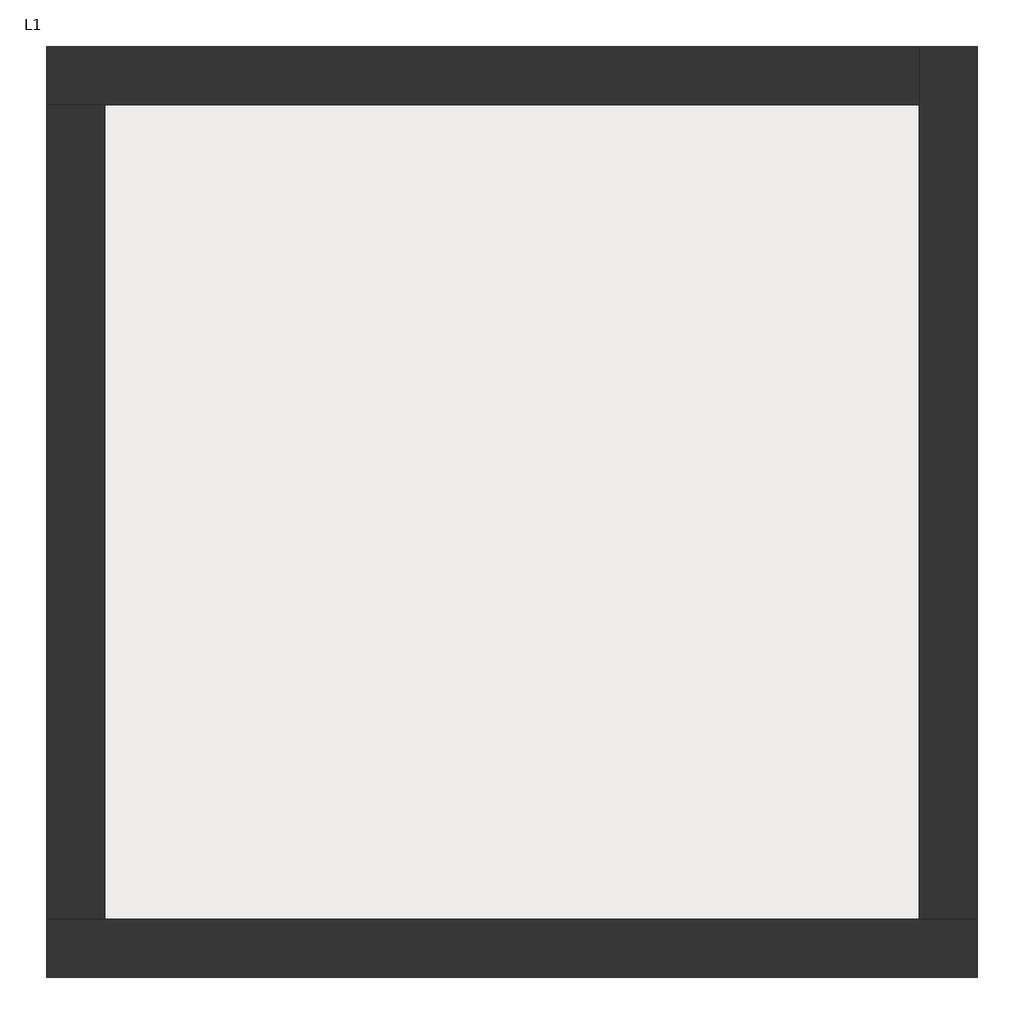
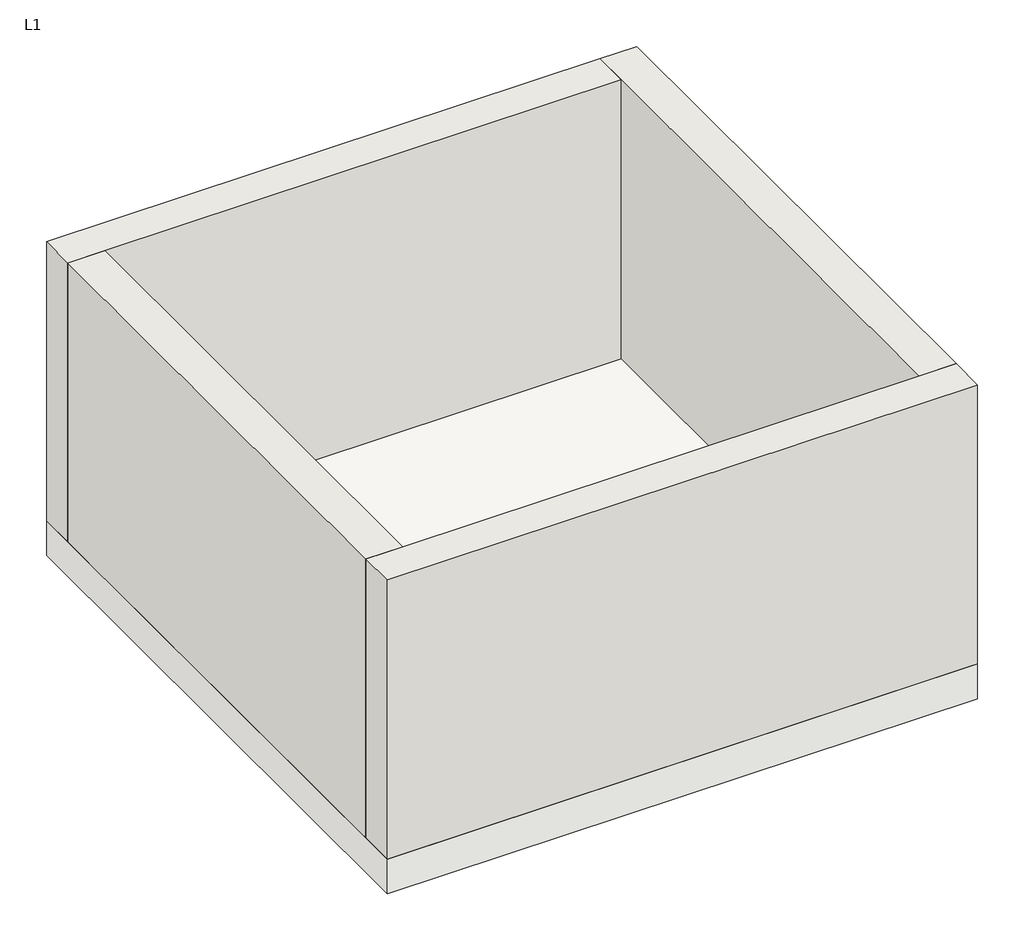
# One storey: 4 walls, 1 slab.
"""IFC4 building model written with IfcOpenShell, lengths in millimetres."""

from ifc_helpers import new_model, si_unit, frame, origin, origin_with_axes, place, context, project, spatial, polyline, outline, extrude, faceted_brep, element, save

model = new_model("IFC4")

# Units and contexts
model_context = context("Model", 3, world=origin())
ifc_project = project(units=[si_unit("LENGTHUNIT", "METRE", prefix="MILLI")], contexts=[model_context])

# Site, building, storey
site = spatial("IfcSite", under=ifc_project)
building = spatial("IfcBuilding", under=site)
storey = spatial("IfcBuildingStorey", under=building, Name="L1", Elevation=0.0)

# Slab
placement = place(None, origin())
element("IfcSlab", 1, ObjectType="FOR INT AC-NH", at=placement, inside=storey, context=model_context, shape_type="SweptSolid", body=[
    extrude(outline(polyline([(0.0, 7999.99416), (7999.99416, 7999.99416), (7999.99416, 0.0), (0.0, 0.0), (0.0, 7999.99416)])), frame((0.0, 0.0, -500.000016), z_axis=(0.0, 0.0, 1.0), x_axis=(1.0, 0.0, 0.0)), (0.0, 0.0, 1.0), 500.000016),
])

# Walls
element("IfcWall", 2, ObjectType="MURO EXTERIOR0.60", at=placement, inside=storey, context=model_context, shape_type="Brep", body=[
    faceted_brep([(0.0, 0.0, 0.0), (7999.99416, 0.0, 0.0), (7999.99416, 0.0, 4000.01232), (0.0, 0.0, 4000.01232), (0.0, 500.000016, 0.0), (0.0, 500.000016, 4000.01232), (500.000016, 500.000016, 4000.01232), (7499.994144, 500.000016, 4000.01232), (7999.99416, 500.000016, 4000.01232), (7999.99416, 500.000016, 0.0), (7499.994144, 500.000016, 0.0), (500.000016, 500.000016, 0.0)], [[[0, 1, 2, 3]], [[4, 5, 6, 7, 8, 9, 10, 11]], [[1, 0, 4, 11, 10, 9]], [[3, 2, 8, 7, 6, 5]], [[2, 1, 9, 8]], [[0, 3, 5, 4]]]),
])
element("IfcWall", 3, ObjectType="MURO EXTERIOR0.60", at=placement, inside=storey, context=model_context, shape_type="Brep", body=[
    faceted_brep([(7999.99416, 500.000016, 0.0), (7999.99416, 7999.99416, 0.0), (7999.99416, 7999.99416, 4000.01232), (7999.99416, 500.000016, 4000.01232), (7499.994144, 500.000016, 0.0), (7499.994144, 500.000016, 4000.01232), (7499.994144, 7499.994144, 4000.01232), (7499.994144, 7999.99416, 4000.01232), (7499.994144, 7999.99416, 0.0), (7499.994144, 7499.994144, 0.0)], [[[0, 1, 2, 3]], [[4, 5, 6, 7, 8, 9]], [[1, 0, 4, 9, 8]], [[3, 2, 7, 6, 5]], [[2, 1, 8, 7]], [[0, 3, 5, 4]]]),
])
element("IfcWall", 4, ObjectType="MURO EXTERIOR0.60", at=placement, inside=storey, context=model_context, shape_type="Brep", body=[
    faceted_brep([(7499.994144, 7999.99416, 0.0), (0.0, 7999.99416, 0.0), (0.0, 7999.99416, 4000.01232), (7499.994144, 7999.99416, 4000.01232), (7499.994144, 7499.994144, 0.0), (7499.994144, 7499.994144, 4000.01232), (500.000016, 7499.994144, 4000.01232), (0.0, 7499.994144, 4000.01232), (0.0, 7499.994144, 0.0), (500.000016, 7499.994144, 0.0)], [[[0, 1, 2, 3]], [[4, 5, 6, 7, 8, 9]], [[1, 0, 4, 9, 8]], [[3, 2, 7, 6, 5]], [[2, 1, 8, 7]], [[0, 3, 5, 4]]]),
])
element("IfcWall", 5, ObjectType="MURO EXTERIOR0.60", at=placement, inside=storey, context=model_context, shape_type="SweptSolid", body=[
    extrude(outline(polyline([(0.0, 500.000016), (0.0, 7499.994144), (500.000016, 7499.994144), (500.000016, 500.000016), (0.0, 500.000016)])), origin_with_axes(), (0.0, 0.0, 1.0), 4000.01232),
])

save(model, "model.ifc")

# Revit data of these elements
# Type "FOR INT AC-NH"
#   Layers, outside or top first: 10 mm no material (function 1); 55 mm no material (function 1); 120 mm no material (function 1); 250 mm no material (function 1); 50 mm no material (function 1); 15 mm no material (function 1)
# Type "MURO EXTERIOR0.60"
#   Description = "Metal Studs with Brick over sheathing on exterior and Gypsum Wall Board (GWB) on interior, Exterior Function"
#   Assembly Code = "B2010158"
#   Type Mark = "W10"
#   Layers, outside or top first: 30 mm no material (function 1); 140 mm no material (function 1); 240 mm no material (function 1); 10 mm no material (function 1); 50 mm no material (function 1); 15 mm no material (function 1); 15 mm no material (function 1)
# Element 1 (IfcSlab, "FOR INT AC-NH")
#   Height Offset From Level = 0 mm
#   Phase Created = New Construction
# Elements 2, 3, 4, 5 (IfcWall, "MURO EXTERIOR0.60")
#   Top Offset = 0 mm
#   Base Offset = 0 mm
#   Unconnected Height = 4000.012 mm
#   wall height = 4000.012 mm
#   Phase Created = New Construction
#   Base Constraint = L1
#   Materials on its faces: "Default Wall"
# Materials
#   "Default Wall": class "Miscellaneous", colour RGB 192 192 192, transparency 0, Cost = 0
